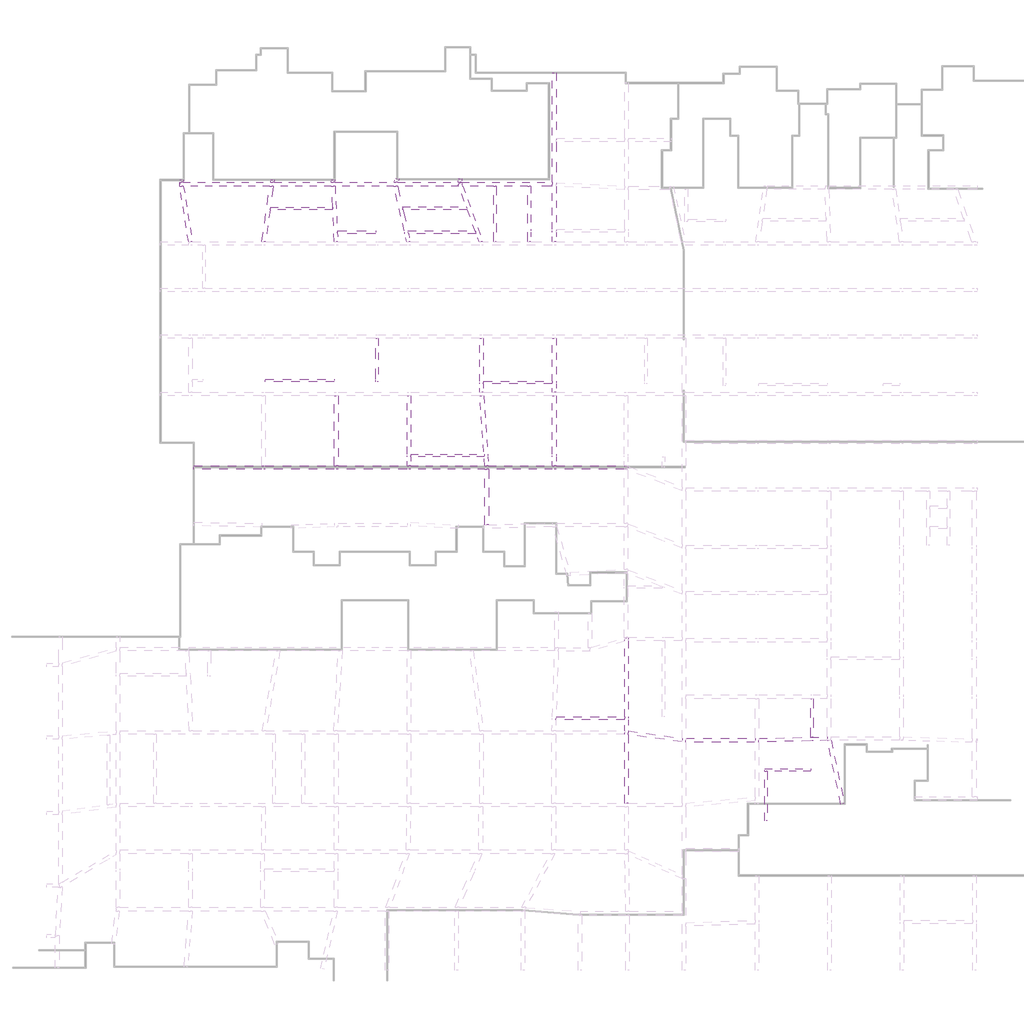
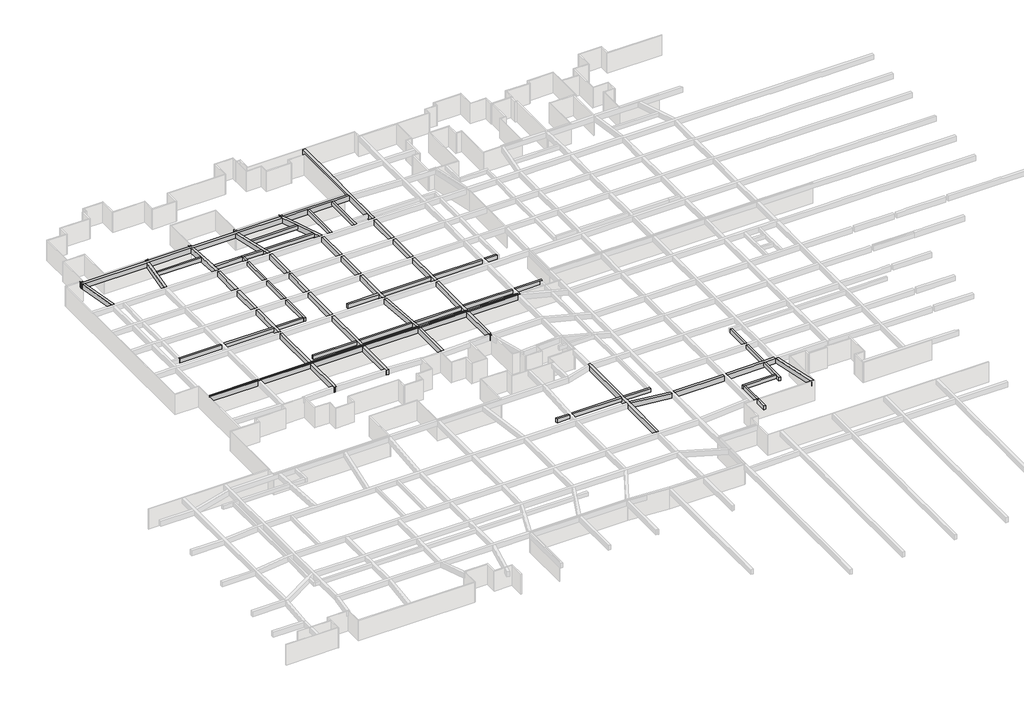
# One storey, part 12 of 16: 40 beams.
"""IFC4 building model written with IfcOpenShell, lengths in millimetres."""

from ifc_helpers import new_model, si_unit, frame, origin, place, context, project, spatial, polyline, outline, extrude, faceted_brep, element, save

model = new_model("IFC4")

# Units and contexts
model_context = context("Model", 3, world=origin())
ifc_project = project(units=[si_unit("LENGTHUNIT", "METRE", prefix="MILLI")], contexts=[model_context])

# Site, building, storey
site = spatial("IfcSite", under=ifc_project)
building = spatial("IfcBuilding", under=site)
storey = spatial("IfcBuildingStorey", under=building, Name="户型图", Elevation=0.0)

# Beams
placement = place(None, origin())
element("IfcBeam", 1, ObjectType="混凝土 - 矩形梁 : KL_beam", at=placement, inside=storey, context=model_context, shape_type="Brep", body=[
    faceted_brep([(86828.9386535, 165312.5884701, 3300.0), (86828.9386535, 165312.5884701, 2500.0), (86828.9386535, 164912.5884701, 2500.0), (86828.9386535, 164912.5884701, 3300.0), (94416.2109037, 164912.5884701, 3300.0), (94816.2109037, 164912.5884701, 3300.0), (102516.2109037, 164912.5884701, 3300.0), (102916.2109037, 164912.5884701, 3300.0), (110616.2109037, 164912.5884701, 3300.0), (111016.2109037, 164912.5884701, 3300.0), (119289.6107616, 164912.5884701, 3300.0), (119689.6107616, 164912.5884701, 3300.0), (126816.2109037, 164912.5884701, 3300.0), (127216.2109037, 164912.5884701, 3300.0), (134828.9386535, 164912.5884701, 3300.0), (134991.8708445, 164912.5884701, 3300.0), (135228.9386535, 164912.5884701, 3300.0), (135228.9386535, 165250.0446618, 3300.0), (135216.2109037, 165254.9303872, 3300.0), (135066.0064625, 165312.5884701, 3300.0), (134816.2109037, 165312.5884701, 3300.0), (127216.2109037, 165312.5884701, 3300.0), (126816.2109037, 165312.5884701, 3300.0), (119676.1137788, 165312.5884701, 3300.0), (119275.1370196, 165312.5884701, 3300.0), (111016.2109037, 165312.5884701, 3300.0), (110616.2109037, 165312.5884701, 3300.0), (102916.2109037, 165312.5884701, 3300.0), (102516.2109037, 165312.5884701, 3300.0), (94816.2109037, 165312.5884701, 3300.0), (94416.2109037, 165312.5884701, 3300.0), (94416.2109037, 164912.5884701, 2500.0), (94816.2109037, 164912.5884701, 2500.0), (102516.2109037, 164912.5884701, 2500.0), (102916.2109037, 164912.5884701, 2500.0), (110616.2109037, 164912.5884701, 2500.0), (111016.2109037, 164912.5884701, 2500.0), (119289.6107616, 164912.5884701, 2500.0), (119689.6107616, 164912.5884701, 2500.0), (126816.2109037, 164912.5884701, 2500.0), (127216.2109037, 164912.5884701, 2500.0), (134828.9386535, 164912.5884701, 2500.0), (134991.8708445, 164912.5884701, 2500.0), (135228.9386535, 164912.5884701, 2500.0), (94416.2109037, 165312.5884701, 2500.0), (94816.2109037, 165312.5884701, 2500.0), (102516.2109037, 165312.5884701, 2500.0), (102916.2109037, 165312.5884701, 2500.0), (110616.2109037, 165312.5884701, 2500.0), (111016.2109037, 165312.5884701, 2500.0), (119275.1370196, 165312.5884701, 2500.0), (119676.1137788, 165312.5884701, 2500.0), (126816.2109037, 165312.5884701, 2500.0), (127216.2109037, 165312.5884701, 2500.0), (134816.2109037, 165312.5884701, 2500.0), (135066.0064625, 165312.5884701, 2500.0), (135216.2109037, 165254.9303872, 2500.0), (135228.9386535, 165250.0446618, 2500.0)], [[[0, 1, 2, 3]], [[0, 3, 4, 5, 6, 7, 8, 9, 10, 11, 12, 13, 14, 15, 16, 17, 18, 19, 20, 21, 22, 23, 24, 25, 26, 27, 28, 29, 30]], [[3, 2, 31, 32, 33, 34, 35, 36, 37, 38, 39, 40, 41, 42, 43, 16, 15, 14, 13, 12, 11, 10, 9, 8, 7, 6, 5, 4]], [[2, 1, 44, 45, 46, 47, 48, 49, 50, 51, 52, 53, 54, 55, 56, 57, 43, 42, 41, 40, 39, 38, 37, 36, 35, 34, 33, 32, 31]], [[1, 0, 30, 29, 28, 27, 26, 25, 24, 23, 22, 21, 20, 19, 55, 54, 53, 52, 51, 50, 49, 48, 47, 46, 45, 44]], [[17, 57, 56, 55, 19, 18]], [[57, 17, 16, 43]]]),
])
element("IfcBeam", 2, ObjectType="混凝土 - 矩形梁 : KL_beam", at=placement, inside=storey, context=model_context, shape_type="Brep", body=[
    faceted_brep([(102916.2109037, 189895.7397162, 3300.0), (102516.2109037, 189895.7397162, 3300.0), (102516.2109037, 185072.5884701, 3300.0), (102916.2109037, 185072.5884701, 3300.0), (102516.2109037, 189895.7397162, 2500.0), (102516.2109037, 185072.5884701, 2500.0), (102916.2109037, 189895.7397162, 2500.0), (102916.2109037, 185072.5884701, 2500.0)], [[[0, 1, 2, 3]], [[1, 4, 5, 2]], [[4, 6, 7, 5]], [[6, 0, 3, 7]], [[1, 0, 6, 4]], [[3, 2, 5, 7]]]),
    faceted_brep([(102516.2109037, 184672.5884701, 3300.0), (102916.2109037, 184672.5884701, 3300.0), (102916.2109037, 184672.5884701, 2500.0), (102516.2109037, 184672.5884701, 2500.0), (102916.2109037, 179912.5884701, 3300.0), (102516.2109037, 179912.5884701, 3300.0), (102516.2109037, 179912.5884701, 2500.0), (102916.2109037, 179912.5884701, 2500.0)], [[[0, 1, 2, 3]], [[4, 5, 6, 7]], [[1, 0, 5, 4]], [[0, 3, 6, 5]], [[3, 2, 7, 6]], [[2, 1, 4, 7]]]),
    faceted_brep([(102916.2109037, 173512.5884701, 3300.0), (102916.2109037, 174669.5403425, 3300.0), (102916.2109037, 174969.5403425, 3300.0), (102916.2109037, 179512.5884701, 3300.0), (102516.2109037, 179512.5884701, 3300.0), (102516.2109037, 174969.5403425, 3300.0), (102516.2109037, 174669.5403425, 3300.0), (102516.2109037, 173512.5884701, 3300.0), (102516.2109037, 179512.5884701, 2500.0), (102516.2109037, 173512.5884701, 2500.0), (102916.2109037, 179512.5884701, 2500.0), (102916.2109037, 173512.5884701, 2500.0)], [[[0, 1, 2, 3, 4, 5, 6, 7]], [[7, 6, 5, 4, 8, 9]], [[9, 8, 10, 11]], [[3, 2, 1, 0, 11, 10]], [[4, 3, 10, 8]], [[0, 7, 9, 11]]]),
    faceted_brep([(102516.2109037, 173112.5884701, 3300.0), (102916.2109037, 173112.5884701, 3300.0), (102916.2109037, 173112.5884701, 2500.0), (102516.2109037, 173112.5884701, 2500.0), (102916.2109037, 165312.5884701, 3300.0), (102516.2109037, 165312.5884701, 3300.0), (102516.2109037, 165312.5884701, 2500.0), (102916.2109037, 165312.5884701, 2500.0)], [[[0, 1, 2, 3]], [[4, 5, 6, 7]], [[1, 0, 5, 4]], [[0, 3, 6, 5]], [[3, 2, 7, 6]], [[2, 1, 4, 7]]]),
    faceted_brep([(102516.2109037, 164912.5884701, 3300.0), (102916.2109037, 164912.5884701, 3300.0), (102916.2109037, 164912.5884701, 2500.0), (102516.2109037, 164912.5884701, 2500.0), (102916.2109037, 158502.9404881, 3300.0), (102719.8772917, 158495.7397162, 3300.0), (102516.2109037, 158488.2700059, 3300.0), (102516.2109037, 158488.2700059, 2500.0), (102719.8772917, 158495.7397162, 2500.0), (102916.2109037, 158502.9404881, 2500.0), (102916.2109037, 158895.7397162, 3300.0), (102516.2109037, 158888.5389443, 3300.0), (102516.2109037, 158888.5389443, 2500.0), (102916.2109037, 158895.7397162, 2500.0)], [[[0, 1, 2, 3]], [[4, 5, 6, 7, 8, 9]], [[6, 5, 4, 10, 1, 0, 11]], [[7, 6, 11, 0, 3, 12]], [[9, 8, 7, 12, 3, 2, 13]], [[4, 9, 13, 2, 1, 10]]]),
])
element("IfcBeam", 3, ObjectType="混凝土 - 矩形梁 : KL_beam", at=placement, inside=storey, context=model_context, shape_type="Brep", body=[
    faceted_brep([(111016.2109037, 189895.7397162, 3300.0), (110616.2109037, 189895.7397162, 3300.0), (110616.2109037, 185072.5884701, 3300.0), (111016.2109037, 185072.5884701, 3300.0), (110616.2109037, 189895.7397162, 2500.0), (110616.2109037, 185072.5884701, 2500.0), (111016.2109037, 189895.7397162, 2500.0), (111016.2109037, 185072.5884701, 2500.0)], [[[0, 1, 2, 3]], [[1, 4, 5, 2]], [[4, 6, 7, 5]], [[6, 0, 3, 7]], [[1, 0, 6, 4]], [[3, 2, 5, 7]]]),
    faceted_brep([(110616.2109037, 184672.5884701, 3300.0), (111016.2109037, 184672.5884701, 3300.0), (111016.2109037, 184672.5884701, 2500.0), (110616.2109037, 184672.5884701, 2500.0), (111016.2109037, 179912.5884701, 3300.0), (110616.2109037, 179912.5884701, 3300.0), (110616.2109037, 179912.5884701, 2500.0), (111016.2109037, 179912.5884701, 2500.0)], [[[0, 1, 2, 3]], [[4, 5, 6, 7]], [[1, 0, 5, 4]], [[0, 3, 6, 5]], [[3, 2, 7, 6]], [[2, 1, 4, 7]]]),
    faceted_brep([(111016.2109037, 179512.5884701, 3300.0), (110616.2109037, 179512.5884701, 3300.0), (110616.2109037, 173512.5884701, 3300.0), (111016.2109037, 173512.5884701, 3300.0), (110616.2109037, 179512.5884701, 2500.0), (110616.2109037, 173512.5884701, 2500.0), (111016.2109037, 179512.5884701, 2500.0), (111016.2109037, 173512.5884701, 2500.0)], [[[0, 1, 2, 3]], [[1, 4, 5, 2]], [[4, 6, 7, 5]], [[6, 0, 3, 7]], [[1, 0, 6, 4]], [[3, 2, 5, 7]]]),
    faceted_brep([(110616.2109037, 173112.5884701, 3300.0), (111016.2109037, 173112.5884701, 3300.0), (111016.2109037, 173112.5884701, 2500.0), (110616.2109037, 173112.5884701, 2500.0), (111016.2109037, 165312.5884701, 3300.0), (110616.2109037, 165312.5884701, 3300.0), (110616.2109037, 165312.5884701, 2500.0), (111016.2109037, 165312.5884701, 2500.0), (110616.2109037, 166595.0298489, 3300.0), (110616.2109037, 166295.0298489, 3300.0), (111016.2109037, 166295.0298489, 3300.0), (111016.2109037, 166595.0298489, 3300.0)], [[[0, 1, 2, 3]], [[4, 5, 6, 7]], [[1, 0, 8, 9, 5, 4, 10, 11]], [[0, 3, 6, 5, 9, 8]], [[3, 2, 7, 6]], [[2, 1, 11, 10, 4, 7]]]),
    faceted_brep([(110616.2109037, 164912.5884701, 3300.0), (111016.2109037, 164912.5884701, 3300.0), (111016.2109037, 164912.5884701, 2500.0), (110616.2109037, 164912.5884701, 2500.0), (111016.2109037, 158495.7397162, 3300.0), (110616.2109037, 158495.7397162, 3300.0), (110616.2109037, 158495.7397162, 2500.0), (111016.2109037, 158495.7397162, 2500.0), (111016.2109037, 158585.1907676, 3300.0), (111016.2109037, 158985.7192923, 3300.0), (110616.2109037, 158895.7397162, 3300.0), (110616.2109037, 158895.7397162, 2500.0), (111016.2109037, 158985.7192923, 2500.0), (111016.2109037, 158585.1907676, 2500.0)], [[[0, 1, 2, 3]], [[4, 5, 6, 7]], [[5, 4, 8, 9, 1, 0, 10]], [[6, 5, 10, 0, 3, 11]], [[7, 6, 11, 3, 2, 12, 13]], [[4, 7, 13, 12, 2, 1, 9, 8]]]),
])
element("IfcBeam", 4, ObjectType="混凝土 - 矩形梁 : KL_beam", at=placement, inside=storey, context=model_context, shape_type="Brep", body=[
    faceted_brep([(118716.2109037, 173512.5884701, 3300.0), (119116.2109037, 173512.5884701, 3300.0), (119116.2109037, 174424.6482986, 3300.0), (119116.2109037, 174724.6482986, 3300.0), (119116.2109037, 179512.5884701, 3300.0), (118716.2109037, 179512.5884701, 3300.0), (118716.2109037, 174724.6482986, 3300.0), (118716.2109037, 174424.6482986, 3300.0), (118716.2109037, 173512.5884701, 2500.0), (118716.2109037, 179512.5884701, 2500.0), (119116.2109037, 173512.5884701, 2500.0), (119116.2109037, 179512.5884701, 2500.0)], [[[0, 1, 2, 3, 4, 5, 6, 7]], [[8, 0, 7, 6, 5, 9]], [[10, 8, 9, 11]], [[1, 10, 11, 4, 3, 2]], [[1, 0, 8, 10]], [[5, 4, 11, 9]]]),
    faceted_brep([(118716.2109037, 189895.7397162, 3300.0), (119116.2109037, 189895.7397162, 3300.0), (119116.2109037, 189895.7397162, 2500.0), (118716.2109037, 189895.7397162, 2500.0), (119116.2109037, 185072.5884701, 3300.0), (118716.2109037, 185072.5884701, 3300.0), (118716.2109037, 185072.5884701, 2500.0), (119116.2109037, 185072.5884701, 2500.0)], [[[0, 1, 2, 3]], [[4, 5, 6, 7]], [[1, 0, 5, 4]], [[0, 3, 6, 5]], [[3, 2, 7, 6]], [[2, 1, 4, 7]]]),
    faceted_brep([(118716.2109037, 184672.5884701, 3300.0), (119116.2109037, 184672.5884701, 3300.0), (119116.2109037, 184672.5884701, 2500.0), (118716.2109037, 184672.5884701, 2500.0), (119116.2109037, 179912.5884701, 3300.0), (118716.2109037, 179912.5884701, 3300.0), (118716.2109037, 179912.5884701, 2500.0), (119116.2109037, 179912.5884701, 2500.0)], [[[0, 1, 2, 3]], [[4, 5, 6, 7]], [[1, 0, 5, 4]], [[0, 3, 6, 5]], [[3, 2, 7, 6]], [[2, 1, 4, 7]]]),
])
element("IfcBeam", 5, ObjectType="混凝土 - 矩形梁 : KL_beam", at=placement, inside=storey, context=model_context, shape_type="Brep", body=[
    faceted_brep([(126816.2109037, 173512.5884701, 3300.0), (127216.2109037, 173512.5884701, 3300.0), (127216.2109037, 174424.6482986, 3300.0), (127216.2109037, 174724.6482986, 3300.0), (127216.2109037, 179512.5884701, 3300.0), (126816.2109037, 179512.5884701, 3300.0), (126816.2109037, 174724.6482986, 3300.0), (126816.2109037, 174424.6482986, 3300.0), (126816.2109037, 173512.5884701, 2500.0), (126816.2109037, 179512.5884701, 2500.0), (127216.2109037, 173512.5884701, 2500.0), (127216.2109037, 179512.5884701, 2500.0)], [[[0, 1, 2, 3, 4, 5, 6, 7]], [[8, 0, 7, 6, 5, 9]], [[10, 8, 9, 11]], [[1, 10, 11, 4, 3, 2]], [[1, 0, 8, 10]], [[5, 4, 11, 9]]]),
    faceted_brep([(126816.2109037, 189895.7397162, 3300.0), (127216.2109037, 189895.7397162, 3300.0), (127216.2109037, 189895.7397162, 2500.0), (126816.2109037, 189895.7397162, 2500.0), (127216.2109037, 185072.5884701, 3300.0), (126816.2109037, 185072.5884701, 3300.0), (126816.2109037, 185072.5884701, 2500.0), (127216.2109037, 185072.5884701, 2500.0)], [[[0, 1, 2, 3]], [[4, 5, 6, 7]], [[1, 0, 5, 4]], [[0, 3, 6, 5]], [[3, 2, 7, 6]], [[2, 1, 4, 7]]]),
    faceted_brep([(126816.2109037, 184672.5884701, 3300.0), (127216.2109037, 184672.5884701, 3300.0), (127216.2109037, 184672.5884701, 2500.0), (126816.2109037, 184672.5884701, 2500.0), (127216.2109037, 179912.5884701, 3300.0), (126816.2109037, 179912.5884701, 3300.0), (126816.2109037, 179912.5884701, 2500.0), (127216.2109037, 179912.5884701, 2500.0)], [[[0, 1, 2, 3]], [[4, 5, 6, 7]], [[1, 0, 5, 4]], [[0, 3, 6, 5]], [[3, 2, 7, 6]], [[2, 1, 4, 7]]]),
])
element("IfcBeam", 6, ObjectType="混凝土 - 矩形梁 : KL_beam", at=placement, inside=storey, context=model_context, shape_type="Brep", body=[
    faceted_brep([(127216.2109037, 173112.5884701, 3300.0), (126816.2109037, 173112.5884701, 3300.0), (126816.2109037, 166595.0298489, 3300.0), (126816.2109037, 166295.0298489, 3300.0), (126816.2109037, 165312.5884701, 3300.0), (127216.2109037, 165312.5884701, 3300.0), (127216.2109037, 166295.0298489, 3300.0), (127216.2109037, 166595.0298489, 3300.0), (126816.2109037, 173112.5884701, 2500.0), (126816.2109037, 165312.5884701, 2500.0), (127216.2109037, 173112.5884701, 2500.0), (127216.2109037, 165312.5884701, 2500.0)], [[[0, 1, 2, 3, 4, 5, 6, 7]], [[1, 8, 9, 4, 3, 2]], [[8, 10, 11, 9]], [[10, 0, 7, 6, 5, 11]], [[1, 0, 10, 8]], [[5, 4, 9, 11]]]),
    faceted_brep([(126816.2109037, 164912.5884701, 3300.0), (127216.2109037, 164912.5884701, 3300.0), (127216.2109037, 164912.5884701, 2500.0), (126816.2109037, 164912.5884701, 2500.0), (126816.2109037, 158509.867597, 3300.0), (126866.6192101, 158511.1605747, 3300.0), (127018.7754912, 158515.0633975, 3300.0), (127216.2109037, 158520.1276342, 3300.0), (127216.2109037, 158915.0633975, 3300.0), (126816.2109037, 158909.9991608, 3300.0), (126816.2109037, 158509.867597, 2500.0), (126816.2109037, 158909.9991608, 2500.0), (127216.2109037, 158520.1276342, 2500.0), (127018.7754912, 158515.0633975, 2500.0), (126866.6192101, 158511.1605747, 2500.0), (127216.2109037, 158915.0633975, 2500.0)], [[[0, 1, 2, 3]], [[4, 5, 6, 7, 8, 1, 0, 9]], [[10, 4, 9, 0, 3, 11]], [[12, 13, 14, 10, 11, 3, 2, 15]], [[7, 12, 15, 2, 1, 8]], [[7, 6, 5, 4, 10, 14, 13, 12]]]),
])
element("IfcBeam", 7, ObjectType="混凝土 - 矩形梁 : KL_beam", at=placement, inside=storey, context=model_context, shape_type="Brep", body=[
    faceted_brep([(119130.6846457, 173112.5884701, 3300.0), (118729.7078864, 173112.5884701, 3300.0), (119185.4599825, 166595.0298489, 3300.0), (119206.4380261, 166295.0298489, 3300.0), (119275.1370196, 165312.5884701, 3300.0), (119676.1137788, 165312.5884701, 3300.0), (119607.4147853, 166295.0298489, 3300.0), (119586.4367417, 166595.0298489, 3300.0), (118729.7078864, 173112.5884701, 2500.0), (119275.1370196, 165312.5884701, 2500.0), (119130.6846457, 173112.5884701, 2500.0), (119676.1137788, 165312.5884701, 2500.0)], [[[0, 1, 2, 3, 4, 5, 6, 7]], [[1, 8, 9, 4, 3, 2]], [[8, 10, 11, 9]], [[10, 0, 7, 6, 5, 11]], [[1, 0, 10, 8]], [[5, 4, 9, 11]]]),
])
element("IfcBeam", 8, ObjectType="混凝土 - 矩形梁 : KL_beam", at=placement, inside=storey, context=model_context, shape_type="Brep", body=[
    faceted_brep([(126816.2109037, 209112.7856546, 3300.0), (127216.2109037, 209112.7856546, 3300.0), (127216.2109037, 209112.7856546, 2500.0), (126816.2109037, 209112.7856546, 2500.0), (126816.2109037, 196873.5880617, 3300.0), (126816.2109037, 196473.5880617, 3300.0), (126816.2109037, 191637.5884701, 3300.0), (126816.2109037, 191337.5884701, 3300.0), (126816.2109037, 190295.7397162, 3300.0), (127216.2109037, 190295.7397162, 3300.0), (127216.2109037, 191337.5884701, 3300.0), (127216.2109037, 191637.5884701, 3300.0), (127216.2109037, 196462.8320366, 3300.0), (127216.2109037, 196863.380975, 3300.0), (127216.2109037, 201412.9009701, 3300.0), (127216.2109037, 201812.9009701, 3300.0), (127216.2109037, 190295.7397162, 2500.0), (127216.2109037, 196462.8320366, 2500.0), (127216.2109037, 196863.380975, 2500.0), (127216.2109037, 201412.9009701, 2500.0), (127216.2109037, 201812.9009701, 2500.0), (126816.2109037, 190295.7397162, 2500.0), (126816.2109037, 196473.5880617, 2500.0), (126816.2109037, 196873.5880617, 2500.0)], [[[0, 1, 2, 3]], [[1, 0, 4, 5, 6, 7, 8, 9, 10, 11, 12, 13, 14, 15]], [[2, 1, 15, 14, 13, 12, 11, 10, 9, 16, 17, 18, 19, 20]], [[3, 2, 20, 19, 18, 17, 16, 21, 22, 23]], [[0, 3, 23, 22, 21, 8, 7, 6, 5, 4]], [[9, 8, 21, 16]]]),
])
element("IfcBeam", 9, ObjectType="混凝土 - 矩形梁 : KL_beam", at=placement, inside=storey, context=model_context, shape_type="Brep", body=[
    faceted_brep([(116662.111408, 196873.5880617, 3300.0), (116286.2343597, 196736.7800043, 3300.0), (116382.0283927, 196473.5880617, 3300.0), (117225.8528022, 194155.1995507, 3300.0), (117335.0438725, 193855.1995507, 3300.0), (118203.3528134, 191469.5403425, 3300.0), (118312.5438836, 191169.5403425, 3300.0), (118630.5813023, 190295.7397162, 3300.0), (119056.2524113, 190295.7397162, 3300.0), (116807.6995017, 196473.5880617, 3300.0), (116662.111408, 196873.5880617, 2500.0), (119056.2524113, 190295.7397162, 2500.0), (116807.6995017, 196473.5880617, 2500.0), (116286.2343597, 196736.7800043, 2500.0), (118630.5813023, 190295.7397162, 2500.0), (116382.0283927, 196473.5880617, 2500.0)], [[[0, 1, 2, 3, 4, 5, 6, 7, 8, 9]], [[10, 0, 9, 8, 11, 12]], [[13, 10, 12, 11, 14, 15]], [[1, 13, 15, 14, 7, 6, 5, 4, 3, 2]], [[8, 7, 14, 11]], [[1, 0, 10, 13]]]),
])
element("IfcBeam", 10, ObjectType="混凝土 - 矩形梁 : KL_beam", at=placement, inside=storey, context=model_context, shape_type="Brep", body=[
    faceted_brep([(116662.111408, 196873.5880617, 3300.0), (116807.6995017, 196473.5880617, 3300.0), (120273.9609037, 196473.5880617, 3300.0), (120573.9609037, 196473.5880617, 3300.0), (124073.9303911, 196473.5880617, 3300.0), (124373.9303911, 196473.5880617, 3300.0), (126816.2109037, 196473.5880617, 3300.0), (126816.2109037, 196873.5880617, 3300.0), (116722.0699004, 196873.5880617, 3300.0), (116807.6995017, 196473.5880617, 2500.0), (126816.2109037, 196473.5880617, 2500.0), (116662.111408, 196873.5880617, 2500.0), (116722.0699004, 196873.5880617, 2500.0), (126816.2109037, 196873.5880617, 2500.0)], [[[0, 1, 2, 3, 4, 5, 6, 7, 8]], [[1, 9, 10, 6, 5, 4, 3, 2]], [[9, 11, 12, 13, 10]], [[11, 0, 8, 7, 13, 12]], [[1, 0, 11, 9]], [[7, 6, 10, 13]]]),
])
element("IfcBeam", 11, ObjectType="混凝土 - 矩形梁 : KL_beam", at=placement, inside=storey, context=model_context, shape_type="Brep", body=[
    faceted_brep([(110564.7764439, 190295.7397162, 3300.0), (110975.298087, 190295.7397162, 3300.0), (110773.565317, 191169.5403425, 3300.0), (110704.3048596, 191469.5403425, 3300.0), (110153.5320336, 193855.1995507, 3300.0), (110084.2715763, 194155.1995507, 3300.0), (109549.0294144, 196473.5880617, 3300.0), (109138.5077713, 196473.5880617, 3300.0), (110293.7832165, 191469.5403425, 3300.0), (110363.0436739, 191169.5403425, 3300.0), (110975.298087, 190295.7397162, 2500.0), (109549.0294144, 196473.5880617, 2500.0), (110564.7764439, 190295.7397162, 2500.0), (109138.5077713, 196473.5880617, 2500.0)], [[[0, 1, 2, 3, 4, 5, 6, 7, 8, 9]], [[1, 10, 11, 6, 5, 4, 3, 2]], [[10, 12, 13, 11]], [[12, 0, 9, 8, 7, 13]], [[1, 0, 12, 10]], [[7, 6, 11, 13]]]),
])
element("IfcBeam", 12, ObjectType="混凝土 - 矩形梁 : KL_beam", at=placement, inside=storey, context=model_context, shape_type="Brep", body=[
    faceted_brep([(116382.0283927, 196473.5880617, 3300.0), (116286.2343597, 196736.7800043, 3300.0), (116662.111408, 196873.5880617, 3300.0), (116322.0699004, 196873.5880617, 3300.0), (109583.224556, 196873.5880617, 3300.0), (109157.553447, 196873.5880617, 3300.0), (102571.4804794, 196873.5880617, 3300.0), (102171.4804794, 196873.5880617, 3300.0), (95823.9296537, 196873.5880617, 3300.0), (95423.9296537, 196873.5880617, 3300.0), (85652.3327458, 196873.5880617, 3300.0), (85281.5166087, 196873.5880617, 3300.0), (85281.5166087, 196473.5880617, 3300.0), (85686.502659, 196473.5880617, 3300.0), (95310.5935192, 196473.5880617, 3300.0), (95714.5245482, 196473.5880617, 3300.0), (102181.6875661, 196473.5880617, 3300.0), (102582.2365045, 196473.5880617, 3300.0), (109138.5077713, 196473.5880617, 3300.0), (109549.0294144, 196473.5880617, 3300.0), (85281.5166087, 196873.5880617, 2500.0), (116662.111408, 196873.5880617, 2500.0), (116322.0699004, 196873.5880617, 2500.0), (109583.224556, 196873.5880617, 2500.0), (109157.553447, 196873.5880617, 2500.0), (102571.4804794, 196873.5880617, 2500.0), (102171.4804794, 196873.5880617, 2500.0), (95823.9296537, 196873.5880617, 2500.0), (95423.9296537, 196873.5880617, 2500.0), (85652.3327458, 196873.5880617, 2500.0), (116286.2343597, 196736.7800043, 2500.0), (116382.0283927, 196473.5880617, 2500.0), (109549.0294144, 196473.5880617, 2500.0), (109138.5077713, 196473.5880617, 2500.0), (102582.2365045, 196473.5880617, 2500.0), (102181.6875661, 196473.5880617, 2500.0), (95714.5245482, 196473.5880617, 2500.0), (95310.5935192, 196473.5880617, 2500.0), (85686.502659, 196473.5880617, 2500.0), (85281.5166087, 196473.5880617, 2500.0)], [[[0, 1, 2, 3, 4, 5, 6, 7, 8, 9, 10, 11, 12, 13, 14, 15, 16, 17, 18, 19]], [[20, 11, 10, 9, 8, 7, 6, 5, 4, 3, 2, 21, 22, 23, 24, 25, 26, 27, 28, 29]], [[30, 31, 32, 33, 34, 35, 36, 37, 38, 39, 20, 29, 28, 27, 26, 25, 24, 23, 22, 21]], [[31, 0, 19, 18, 17, 16, 15, 14, 13, 12, 39, 38, 37, 36, 35, 34, 33, 32]], [[1, 0, 31, 30]], [[12, 11, 20, 39]], [[1, 30, 21, 2]]]),
])
element("IfcBeam", 13, ObjectType="混凝土 - 矩形梁 : KL_beam", at=placement, inside=storey, context=model_context, shape_type="Brep", body=[
    faceted_brep([(94442.3535561, 190295.7397162, 3300.0), (94846.2845851, 190295.7397162, 3300.0), (95341.1878431, 193817.1593735, 3300.0), (95383.3500935, 194117.1593735, 3300.0), (95714.5245482, 196473.5880617, 3300.0), (95310.5935192, 196473.5880617, 3300.0), (94846.2845851, 190295.7397162, 2500.0), (95714.5245482, 196473.5880617, 2500.0), (94442.3535561, 190295.7397162, 2500.0), (95310.5935192, 196473.5880617, 2500.0)], [[[0, 1, 2, 3, 4, 5]], [[1, 6, 7, 4, 3, 2]], [[6, 8, 9, 7]], [[8, 0, 5, 9]], [[1, 0, 8, 6]], [[5, 4, 7, 9]]]),
])
element("IfcBeam", 14, ObjectType="混凝土 - 矩形梁 : KL_beam", at=placement, inside=storey, context=model_context, shape_type="Brep", body=[
    faceted_brep([(102505.4548786, 190295.7397162, 3300.0), (102906.003817, 190295.7397162, 3300.0), (102860.2098666, 191169.5403425, 3300.0), (102844.4875329, 191469.5403425, 3300.0), (102582.2365045, 196473.5880617, 3300.0), (102181.6875661, 196473.5880617, 3300.0), (102305.1827607, 194117.1593735, 3300.0), (102320.9050944, 193817.1593735, 3300.0), (102906.003817, 190295.7397162, 2500.0), (102582.2365045, 196473.5880617, 2500.0), (102505.4548786, 190295.7397162, 2500.0), (102181.6875661, 196473.5880617, 2500.0)], [[[0, 1, 2, 3, 4, 5, 6, 7]], [[1, 8, 9, 4, 3, 2]], [[8, 10, 11, 9]], [[10, 0, 7, 6, 5, 11]], [[1, 0, 10, 8]], [[5, 4, 9, 11]]]),
])
element("IfcBeam", 15, ObjectType="混凝土 - 矩形梁 : KL_beam", at=placement, inside=storey, context=model_context, shape_type="Brep", body=[
    faceted_brep([(86259.9916613, 190295.7397162, 3300.0), (86294.1615746, 190295.7397162, 3300.0), (86664.9777116, 190295.7397162, 3300.0), (85686.502659, 196473.5880617, 3300.0), (85281.5166087, 196473.5880617, 3300.0), (86664.9777116, 190295.7397162, 2500.0), (85686.502659, 196473.5880617, 2500.0), (86294.1615746, 190295.7397162, 2500.0), (86259.9916613, 190295.7397162, 2500.0), (85281.5166087, 196473.5880617, 2500.0)], [[[0, 1, 2, 3, 4]], [[2, 5, 6, 3]], [[5, 7, 8, 9, 6]], [[8, 0, 4, 9]], [[5, 2, 1, 0, 8, 7]], [[4, 3, 6, 9]]]),
])
element("IfcBeam", 16, ObjectType="混凝土 - 矩形梁 : KL_beam", at=placement, inside=storey, context=model_context, shape_type="Brep", body=[
    faceted_brep([(85252.3327458, 197173.5880617, 3300.0), (85652.3327458, 197173.5880617, 3300.0), (85652.3327458, 197173.5880617, 2500.0), (85252.3327458, 197173.5880617, 2500.0), (85252.3327458, 196657.8477203, 3300.0), (85281.5166087, 196473.5880617, 3300.0), (85281.5166087, 196873.5880617, 3300.0), (85623.1488829, 196873.5880617, 3300.0), (85652.3327458, 196873.5880617, 3300.0), (85652.3327458, 196873.5880617, 2500.0), (85623.1488829, 196873.5880617, 2500.0), (85281.5166087, 196873.5880617, 2500.0), (85281.5166087, 196473.5880617, 2500.0), (85252.3327458, 196657.8477203, 2500.0)], [[[0, 1, 2, 3]], [[1, 0, 4, 5, 6, 7, 8]], [[2, 1, 8, 9]], [[3, 2, 9, 10, 11, 12, 13]], [[0, 3, 13, 4]], [[5, 4, 13, 12]], [[6, 11, 10, 9, 8, 7]], [[11, 6, 5, 12]]]),
])
element("IfcBeam", 17, ObjectType="混凝土 - 矩形梁 : KL_beam", at=placement, inside=storey, context=model_context, shape_type="SweptSolid", body=[
    extrude(outline(polyline([(95423.9296537, 197162.7132659), (95823.9296537, 197162.7132659), (95823.9296537, 196873.5880617), (95423.9296537, 196873.5880617), (95423.9296537, 197162.7132659)])), frame((0.0, 0.0, 2500.0), z_axis=(0.0, 0.0, 1.0), x_axis=(1.0, 0.0, 0.0)), (0.0, 0.0, 1.0), 800.0),
])
element("IfcBeam", 18, ObjectType="混凝土 - 矩形梁 : KL_beam", at=placement, inside=storey, context=model_context, shape_type="SweptSolid", body=[
    extrude(outline(polyline([(102171.4804794, 197162.7132659), (102571.4804794, 197162.7132659), (102571.4804794, 196873.5880617), (102171.4804794, 196873.5880617), (102171.4804794, 197162.7132659)])), frame((0.0, 0.0, 2500.0), z_axis=(0.0, 0.0, 1.0), x_axis=(1.0, 0.0, 0.0)), (0.0, 0.0, 1.0), 800.0),
])
element("IfcBeam", 19, ObjectType="混凝土 - 矩形梁 : KL_beam", at=placement, inside=storey, context=model_context, shape_type="SweptSolid", body=[
    extrude(outline(polyline([(109335.8848749, 197363.5496329), (109711.7619232, 197226.7415756), (109583.224556, 196873.5880617), (109157.553447, 196873.5880617), (109335.8848749, 197363.5496329)])), frame((0.0, 0.0, 2500.0), z_axis=(0.0, 0.0, 1.0), x_axis=(1.0, 0.0, 0.0)), (0.0, 0.0, 1.0), 800.0),
])
element("IfcBeam", 20, ObjectType="混凝土 - 矩形梁 : KL_beam", at=placement, inside=storey, context=model_context, shape_type="Brep", body=[
    faceted_brep([(116322.0699004, 197262.7098479, 3300.0), (116722.0699004, 197262.7098479, 3300.0), (116722.0699004, 197262.7098479, 2500.0), (116322.0699004, 197262.7098479, 2500.0), (116322.0699004, 196873.5880617, 3300.0), (116662.111408, 196873.5880617, 3300.0), (116722.0699004, 196873.5880617, 3300.0), (116722.0699004, 196873.5880617, 2500.0), (116662.111408, 196873.5880617, 2500.0), (116322.0699004, 196873.5880617, 2500.0)], [[[0, 1, 2, 3]], [[1, 0, 4, 5, 6]], [[2, 1, 6, 7]], [[3, 2, 7, 8, 9]], [[0, 3, 9, 4]], [[4, 9, 8, 7, 6, 5]]]),
])
element("IfcBeam", 21, ObjectType="混凝土 - 矩形梁 : KL_beam", at=placement, inside=storey, context=model_context, shape_type="SweptSolid", body=[
    extrude(outline(polyline([(119289.6107616, 164912.5884701), (119689.6107616, 164912.5884701), (119689.6107616, 158727.2012041), (119289.6107616, 158716.9411668), (119289.6107616, 164912.5884701)])), frame((0.0, 0.0, 2500.0), z_axis=(0.0, 0.0, 1.0), x_axis=(1.0, 0.0, 0.0)), (0.0, 0.0, 1.0), 800.0),
])
element("IfcBeam", 22, ObjectType="混凝土 - 矩形梁 : KL_beam", at=placement, inside=storey, context=model_context, shape_type="SweptSolid", body=[
    extrude(outline(polyline([(141666.2091209, 134512.5884701), (141666.2091209, 134912.5884701), (149416.2109037, 134912.5884701), (149416.2109037, 134512.5884701), (141666.2091209, 134512.5884701)])), frame((0.0, 0.0, 2500.0), z_axis=(0.0, 0.0, 1.0), x_axis=(1.0, 0.0, 0.0)), (0.0, 0.0, 1.0), 800.0),
])
element("IfcBeam", 23, ObjectType="混凝土 - 矩形梁 : KL_beam", at=placement, inside=storey, context=model_context, shape_type="Brep", body=[
    faceted_brep([(157416.2109037, 134691.1376184, 3300.0), (157416.2109037, 135091.241133, 3300.0), (155875.8505966, 135056.1953134, 3300.0), (155575.8505966, 135049.3698027, 3300.0), (149816.2109037, 134918.3281936, 3300.0), (149816.2109037, 134518.224679, 3300.0), (155575.8505966, 134649.2662881, 3300.0), (155875.8505966, 134656.0917988, 3300.0), (157416.2109037, 134691.1376184, 2500.0), (149816.2109037, 134518.224679, 2500.0), (157416.2109037, 135091.241133, 2500.0), (149816.2109037, 134918.3281936, 2500.0)], [[[0, 1, 2, 3, 4, 5, 6, 7]], [[8, 0, 7, 6, 5, 9]], [[10, 8, 9, 11]], [[1, 10, 11, 4, 3, 2]], [[1, 0, 8, 10]], [[4, 11, 9, 5]]]),
])
element("IfcBeam", 24, ObjectType="混凝土 - 矩形梁 : KL_beam", at=placement, inside=storey, context=model_context, shape_type="SweptSolid", body=[
    extrude(outline(polyline([(159354.4261806, 127680.0266564), (158963.1671403, 127596.86198), (157455.0445029, 134692.0211489), (157618.4857796, 134695.7397162), (157863.190335, 134695.7397162), (159354.4261806, 127680.0266564)])), frame((0.0, 0.0, 2500.0), z_axis=(0.0, 0.0, 1.0), x_axis=(1.0, 0.0, 0.0)), (0.0, 0.0, 1.0), 800.0),
])
element("IfcBeam", 25, ObjectType="混凝土 - 矩形梁 : KL_beam", at=placement, inside=storey, context=model_context, shape_type="SweptSolid", body=[
    extrude(outline(polyline([(141266.2091209, 134941.3479482), (141266.2091209, 134537.7323272), (135272.1367776, 135345.4835538), (135272.1367776, 135749.0991749), (141266.2091209, 134941.3479482)])), frame((0.0, 0.0, 2500.0), z_axis=(0.0, 0.0, 1.0), x_axis=(1.0, 0.0, 0.0)), (0.0, 0.0, 1.0), 800.0),
])
element("IfcBeam", 26, ObjectType="混凝土 - 矩形梁 : KL_beam", at=placement, inside=storey, context=model_context, shape_type="Brep", body=[
    faceted_brep([(135272.1367776, 146146.9200065, 3300.0), (134872.1367776, 146146.9200065, 3300.0), (134872.1367776, 145730.5761084, 3300.0), (134872.1367776, 137322.9773199, 3300.0), (134872.1367776, 137022.9773199, 3300.0), (134872.1367776, 135771.3777961, 3300.0), (134872.1367776, 135371.3777961, 3300.0), (134872.1367776, 127693.5189202, 3300.0), (135272.1367776, 127693.5189202, 3300.0), (135272.1367776, 135345.4835538, 3300.0), (135272.1367776, 135749.0991749, 3300.0), (135272.1367776, 137022.9773199, 3300.0), (135272.1367776, 137322.9773199, 3300.0), (135272.1367776, 145796.5023677, 3300.0), (134872.1367776, 146146.9200065, 2500.0), (134872.1367776, 145730.5761084, 2500.0), (134872.1367776, 135771.3777961, 2500.0), (134872.1367776, 135371.3777961, 2500.0), (134872.1367776, 127693.5189202, 2500.0), (135272.1367776, 146146.9200065, 2500.0), (135272.1367776, 145796.5023677, 2500.0), (135272.1367776, 135749.0991749, 2500.0), (135272.1367776, 135345.4835538, 2500.0), (135272.1367776, 127693.5189202, 2500.0)], [[[0, 1, 2, 3, 4, 5, 6, 7, 8, 9, 10, 11, 12, 13]], [[1, 14, 15, 16, 17, 18, 7, 6, 5, 4, 3, 2]], [[14, 19, 20, 21, 22, 23, 18, 17, 16, 15]], [[19, 0, 13, 12, 11, 10, 9, 8, 23, 22, 21, 20]], [[8, 7, 18, 23]], [[0, 19, 14, 1]]]),
])
element("IfcBeam", 27, ObjectType="混凝土 - 矩形梁 : L_beam", at=placement, inside=storey, context=model_context, shape_type="SweptSolid", body=[
    extrude(outline(polyline([(95341.1878431, 193817.1593735), (95383.3500935, 194117.1593735), (102305.1827607, 194117.1593735), (102320.9050944, 193817.1593735), (95341.1878431, 193817.1593735)])), frame((0.0, 0.0, 2700.0), z_axis=(0.0, 0.0, 1.0), x_axis=(1.0, 0.0, 0.0)), (0.0, 0.0, 1.0), 600.0),
])
element("IfcBeam", 28, ObjectType="混凝土 - 矩形梁 : L_beam", at=placement, inside=storey, context=model_context, shape_type="SweptSolid", body=[
    extrude(outline(polyline([(117225.8528022, 194155.1995507), (117335.0438725, 193855.1995507), (110153.5320336, 193855.1995507), (110084.2715763, 194155.1995507), (117225.8528022, 194155.1995507)])), frame((0.0, 0.0, 2700.0), z_axis=(0.0, 0.0, 1.0), x_axis=(1.0, 0.0, 0.0)), (0.0, 0.0, 1.0), 600.0),
])
element("IfcBeam", 29, ObjectType="混凝土 - 矩形梁 : L_beam", at=placement, inside=storey, context=model_context, shape_type="SweptSolid", body=[
    extrude(outline(polyline([(120573.9609037, 190295.7397162), (120273.9609037, 190295.7397162), (120273.9609037, 196473.5880617), (120573.9609037, 196473.5880617), (120573.9609037, 190295.7397162)])), frame((0.0, 0.0, 2700.0), z_axis=(0.0, 0.0, 1.0), x_axis=(1.0, 0.0, 0.0)), (0.0, 0.0, 1.0), 600.0),
])
element("IfcBeam", 30, ObjectType="混凝土 - 矩形梁 : L_beam", at=placement, inside=storey, context=model_context, shape_type="Brep", body=[
    faceted_brep([(124073.9303911, 190295.7397162, 3300.0), (124373.9303911, 190295.7397162, 3300.0), (124373.9303911, 191337.5884701, 3300.0), (124373.9303911, 191637.5884701, 3300.0), (124373.9303911, 196473.5880617, 3300.0), (124073.9303911, 196473.5880617, 3300.0), (124073.9303911, 190295.7397162, 2700.0), (124073.9303911, 196473.5880617, 2700.0), (124373.9303911, 190295.7397162, 2700.0), (124373.9303911, 196473.5880617, 2700.0), (124373.9303911, 191637.5884701, 2700.0), (124373.9303911, 191337.5884701, 2700.0)], [[[0, 1, 2, 3, 4, 5]], [[6, 0, 5, 7]], [[8, 6, 7, 9, 10, 11]], [[1, 8, 11, 10, 9, 4, 3, 2]], [[1, 0, 6, 8]], [[5, 4, 9, 7]]]),
])
element("IfcBeam", 31, ObjectType="混凝土 - 矩形梁 : L_beam", at=placement, inside=storey, context=model_context, shape_type="Brep", body=[
    faceted_brep([(107120.783903, 191469.5403425, 3300.0), (107120.783903, 191169.5403425, 3300.0), (107420.783903, 191169.5403425, 3300.0), (110363.0436739, 191169.5403425, 3300.0), (110293.7832165, 191469.5403425, 3300.0), (107120.783903, 191469.5403425, 2700.0), (110293.7832165, 191469.5403425, 2700.0), (107120.783903, 191169.5403425, 2700.0), (110363.0436739, 191169.5403425, 2700.0), (107420.783903, 191169.5403425, 2700.0)], [[[0, 1, 2, 3, 4]], [[5, 0, 4, 6]], [[7, 5, 6, 8, 9]], [[1, 7, 9, 8, 3, 2]], [[4, 3, 8, 6]], [[1, 0, 5, 7]]]),
    faceted_brep([(118203.3528134, 191469.5403425, 3300.0), (118312.5438836, 191169.5403425, 3300.0), (118312.5438836, 191169.5403425, 2700.0), (118203.3528134, 191469.5403425, 2700.0), (110773.565317, 191169.5403425, 3300.0), (110704.3048596, 191469.5403425, 3300.0), (110704.3048596, 191469.5403425, 2700.0), (110773.565317, 191169.5403425, 2700.0)], [[[0, 1, 2, 3]], [[4, 5, 6, 7]], [[1, 0, 5, 4]], [[0, 3, 6, 5]], [[3, 2, 7, 6]], [[2, 1, 4, 7]]]),
])
element("IfcBeam", 32, ObjectType="混凝土 - 矩形梁 : L_beam", at=placement, inside=storey, context=model_context, shape_type="Brep", body=[
    faceted_brep([(107120.783903, 174669.5403425, 3300.0), (107420.783903, 174669.5403425, 3300.0), (107420.783903, 179512.5884701, 3300.0), (107120.783903, 179512.5884701, 3300.0), (107120.783903, 174969.5403425, 3300.0), (107120.783903, 174669.5403425, 2700.0), (107120.783903, 179512.5884701, 2700.0), (107120.783903, 174969.5403425, 2700.0), (107420.783903, 174669.5403425, 2700.0), (107420.783903, 179512.5884701, 2700.0)], [[[0, 1, 2, 3, 4]], [[5, 0, 4, 3, 6, 7]], [[8, 5, 7, 6, 9]], [[1, 8, 9, 2]], [[3, 2, 9, 6]], [[1, 0, 5, 8]]]),
    faceted_brep([(107120.783903, 191169.5403425, 3300.0), (107420.783903, 191169.5403425, 3300.0), (107420.783903, 191169.5403425, 2700.0), (107120.783903, 191169.5403425, 2700.0), (107420.783903, 190295.7397162, 3300.0), (107120.783903, 190295.7397162, 3300.0), (107120.783903, 190295.7397162, 2700.0), (107420.783903, 190295.7397162, 2700.0)], [[[0, 1, 2, 3]], [[4, 5, 6, 7]], [[1, 0, 5, 4]], [[0, 3, 6, 5]], [[3, 2, 7, 6]], [[2, 1, 4, 7]]]),
    faceted_brep([(107120.783903, 189895.7397162, 3300.0), (107420.783903, 189895.7397162, 3300.0), (107420.783903, 189895.7397162, 2700.0), (107120.783903, 189895.7397162, 2700.0), (107420.783903, 185072.5884701, 3300.0), (107120.783903, 185072.5884701, 3300.0), (107120.783903, 185072.5884701, 2700.0), (107420.783903, 185072.5884701, 2700.0)], [[[0, 1, 2, 3]], [[4, 5, 6, 7]], [[1, 0, 5, 4]], [[0, 3, 6, 5]], [[3, 2, 7, 6]], [[2, 1, 4, 7]]]),
    faceted_brep([(107120.783903, 184672.5884701, 3300.0), (107420.783903, 184672.5884701, 3300.0), (107420.783903, 184672.5884701, 2700.0), (107120.783903, 184672.5884701, 2700.0), (107420.783903, 179912.5884701, 3300.0), (107120.783903, 179912.5884701, 3300.0), (107120.783903, 179912.5884701, 2700.0), (107420.783903, 179912.5884701, 2700.0)], [[[0, 1, 2, 3]], [[4, 5, 6, 7]], [[1, 0, 5, 4]], [[0, 3, 6, 5]], [[3, 2, 7, 6]], [[2, 1, 4, 7]]]),
])
element("IfcBeam", 33, ObjectType="混凝土 - 矩形梁 : L_beam", at=placement, inside=storey, context=model_context, shape_type="Brep", body=[
    faceted_brep([(107120.783903, 174669.5403425, 3300.0), (107120.783903, 174969.5403425, 3300.0), (102916.2109037, 174969.5403425, 3300.0), (102916.2109037, 174669.5403425, 3300.0), (107120.783903, 174969.5403425, 2700.0), (102916.2109037, 174969.5403425, 2700.0), (107120.783903, 174669.5403425, 2700.0), (102916.2109037, 174669.5403425, 2700.0)], [[[0, 1, 2, 3]], [[1, 4, 5, 2]], [[4, 6, 7, 5]], [[6, 0, 3, 7]], [[1, 0, 6, 4]], [[3, 2, 5, 7]]]),
    faceted_brep([(94416.2109037, 174969.5403425, 3300.0), (94416.2109037, 174669.5403425, 3300.0), (94416.2109037, 174669.5403425, 2700.0), (94416.2109037, 174969.5403425, 2700.0), (88120.783903, 174969.5403425, 3300.0), (87820.783903, 174969.5403425, 3300.0), (87820.783903, 174669.5403425, 3300.0), (88120.783903, 174969.5403425, 2700.0), (87820.783903, 174969.5403425, 2700.0), (87820.783903, 174669.5403425, 2700.0)], [[[0, 1, 2, 3]], [[1, 0, 4, 5, 6]], [[0, 3, 7, 8, 5, 4]], [[3, 2, 9, 8, 7]], [[2, 1, 6, 9]], [[6, 5, 8, 9]]]),
    faceted_brep([(94816.2109037, 174669.5403425, 3300.0), (94816.2109037, 174969.5403425, 3300.0), (94816.2109037, 174969.5403425, 2700.0), (94816.2109037, 174669.5403425, 2700.0), (102516.2109037, 174969.5403425, 3300.0), (102516.2109037, 174669.5403425, 3300.0), (102516.2109037, 174669.5403425, 2700.0), (102516.2109037, 174969.5403425, 2700.0)], [[[0, 1, 2, 3]], [[4, 5, 6, 7]], [[1, 0, 5, 4]], [[2, 1, 4, 7]], [[3, 2, 7, 6]], [[0, 3, 6, 5]]]),
])
element("IfcBeam", 34, ObjectType="混凝土 - 矩形梁 : L_beam", at=placement, inside=storey, context=model_context, shape_type="SweptSolid", body=[
    extrude(outline(polyline([(107120.783903, 191469.5403425), (107120.783903, 191169.5403425), (102860.2098666, 191169.5403425), (102844.4875329, 191469.5403425), (107120.783903, 191469.5403425)])), frame((0.0, 0.0, 2700.0), z_axis=(0.0, 0.0, 1.0), x_axis=(1.0, 0.0, 0.0)), (0.0, 0.0, 1.0), 600.0),
])
element("IfcBeam", 35, ObjectType="混凝土 - 矩形梁 : L_beam", at=placement, inside=storey, context=model_context, shape_type="SweptSolid", body=[
    extrude(outline(polyline([(113817.7397943, 174424.6482986), (113817.7397943, 174724.6482986), (118716.2109037, 174724.6482986), (118716.2109037, 174424.6482986), (113817.7397943, 174424.6482986)])), frame((0.0, 0.0, 2700.0), z_axis=(0.0, 0.0, 1.0), x_axis=(1.0, 0.0, 0.0)), (0.0, 0.0, 1.0), 600.0),
    extrude(outline(polyline([(137101.0841862, 174724.6482986), (137101.0841862, 174424.6482986), (135216.2109037, 174424.6482986), (135216.2109037, 174724.6482986), (137101.0841862, 174724.6482986)])), frame((0.0, 0.0, 2700.0), z_axis=(0.0, 0.0, 1.0), x_axis=(1.0, 0.0, 0.0)), (0.0, 0.0, 1.0), 600.0),
    extrude(outline(polyline([(119116.2109037, 174424.6482986), (119116.2109037, 174724.6482986), (126816.2109037, 174724.6482986), (126816.2109037, 174424.6482986), (119116.2109037, 174424.6482986)])), frame((0.0, 0.0, 2700.0), z_axis=(0.0, 0.0, 1.0), x_axis=(1.0, 0.0, 0.0)), (0.0, 0.0, 1.0), 600.0),
    extrude(outline(polyline([(127216.2109037, 174424.6482986), (127216.2109037, 174724.6482986), (134816.2109037, 174724.6482986), (134816.2109037, 174424.6482986), (127216.2109037, 174424.6482986)])), frame((0.0, 0.0, 2700.0), z_axis=(0.0, 0.0, 1.0), x_axis=(1.0, 0.0, 0.0)), (0.0, 0.0, 1.0), 600.0),
])
element("IfcBeam", 36, ObjectType="混凝土 - 矩形梁 : L_beam", at=placement, inside=storey, context=model_context, shape_type="Brep", body=[
    faceted_brep([(155875.8505966, 130545.9909389, 3300.0), (155575.8505966, 130545.9909389, 3300.0), (155575.8505966, 130545.9909389, 2700.0), (155875.8505966, 130545.9909389, 2700.0), (155875.8505966, 134656.0917988, 3300.0), (155575.8505966, 134649.2662881, 3300.0), (155575.8505966, 131538.0259701, 3300.0), (155575.8505966, 131238.0259701, 3300.0), (155575.8505966, 134649.2662881, 2700.0), (155575.8505966, 131538.0259701, 2700.0), (155575.8505966, 131238.0259701, 2700.0), (155875.8505966, 134656.0917988, 2700.0)], [[[0, 1, 2, 3]], [[1, 0, 4, 5, 6, 7]], [[2, 1, 7, 6, 5, 8, 9, 10]], [[3, 2, 10, 9, 8, 11]], [[0, 3, 11, 4]], [[5, 4, 11, 8]]]),
    faceted_brep([(155575.8505966, 143695.3207545, 3300.0), (155875.8505966, 143695.3207545, 3300.0), (155875.8505966, 143695.3207545, 2700.0), (155575.8505966, 143695.3207545, 2700.0), (155875.8505966, 139762.5884701, 3300.0), (155575.8505966, 139762.5884701, 3300.0), (155575.8505966, 139762.5884701, 2700.0), (155875.8505966, 139762.5884701, 2700.0)], [[[0, 1, 2, 3]], [[4, 5, 6, 7]], [[1, 0, 5, 4]], [[0, 3, 6, 5]], [[3, 2, 7, 6]], [[2, 1, 4, 7]]]),
    faceted_brep([(155575.8505966, 139362.5884701, 3300.0), (155875.8505966, 139362.5884701, 3300.0), (155875.8505966, 139362.5884701, 2700.0), (155575.8505966, 139362.5884701, 2700.0), (155875.8505966, 135056.1953134, 3300.0), (155575.8505966, 135049.3698027, 3300.0), (155575.8505966, 135049.3698027, 2700.0), (155875.8505966, 135056.1953134, 2700.0)], [[[0, 1, 2, 3]], [[4, 5, 6, 7]], [[1, 0, 5, 4]], [[0, 3, 6, 5]], [[3, 2, 7, 6]], [[2, 1, 4, 7]]]),
])
element("IfcBeam", 37, ObjectType="混凝土 - 矩形梁 : L_beam", at=placement, inside=storey, context=model_context, shape_type="Brep", body=[
    faceted_brep([(150475.8505966, 131538.0259701, 3300.0), (150475.8505966, 131238.0259701, 3300.0), (150775.8505966, 131238.0259701, 3300.0), (155575.8505966, 131238.0259701, 3300.0), (155575.8505966, 131538.0259701, 3300.0), (150475.8505966, 131538.0259701, 2700.0), (155575.8505966, 131538.0259701, 2700.0), (150475.8505966, 131238.0259701, 2700.0), (155575.8505966, 131238.0259701, 2700.0), (150775.8505966, 131238.0259701, 2700.0)], [[[0, 1, 2, 3, 4]], [[5, 0, 4, 6]], [[7, 5, 6, 8, 9]], [[1, 7, 9, 8, 3, 2]], [[4, 3, 8, 6]], [[1, 0, 5, 7]]]),
])
element("IfcBeam", 38, ObjectType="混凝土 - 矩形梁 : L_beam", at=placement, inside=storey, context=model_context, shape_type="SweptSolid", body=[
    extrude(outline(polyline([(150775.8505966, 125740.9123315), (150475.8505966, 125740.9123315), (150475.8505966, 131238.0259701), (150775.8505966, 131238.0259701), (150775.8505966, 125740.9123315)])), frame((0.0, 0.0, 2700.0), z_axis=(0.0, 0.0, 1.0), x_axis=(1.0, 0.0, 0.0)), (0.0, 0.0, 1.0), 600.0),
])
element("IfcBeam", 39, ObjectType="混凝土 - 矩形梁 : L_beam", at=placement, inside=storey, context=model_context, shape_type="Brep", body=[
    faceted_brep([(124805.6772345, 137322.9773199, 3300.0), (124805.6772345, 137322.9773199, 2700.0), (124805.6772345, 137022.9773199, 2700.0), (124805.6772345, 137022.9773199, 3300.0), (126813.4099874, 137322.9773199, 3300.0), (126802.9337565, 137022.9773199, 3300.0), (126802.9337565, 137022.9773199, 2700.0), (126813.4099874, 137322.9773199, 2700.0)], [[[0, 1, 2, 3]], [[4, 5, 6, 7]], [[0, 3, 5, 4]], [[3, 2, 6, 5]], [[2, 1, 7, 6]], [[1, 0, 4, 7]]]),
    faceted_brep([(127213.6538051, 137322.9773199, 3300.0), (127203.1775743, 137022.9773199, 3300.0), (134872.1367776, 137022.9773199, 3300.0), (134872.1367776, 137322.9773199, 3300.0), (127203.1775743, 137022.9773199, 2700.0), (134872.1367776, 137022.9773199, 2700.0), (127213.6538051, 137322.9773199, 2700.0), (134872.1367776, 137322.9773199, 2700.0)], [[[0, 1, 2, 3]], [[1, 4, 5, 2]], [[4, 6, 7, 5]], [[6, 0, 3, 7]], [[1, 0, 6, 4]], [[3, 2, 5, 7]]]),
    faceted_brep([(135272.1367776, 137022.9773199, 3300.0), (135272.1367776, 137322.9773199, 3300.0), (135272.1367776, 137322.9773199, 2700.0), (135272.1367776, 137022.9773199, 2700.0), (139349.0511844, 137022.9773199, 3300.0), (139349.0511844, 137322.9773199, 3300.0), (139049.0511844, 137322.9773199, 3300.0), (139349.0511844, 137022.9773199, 2700.0), (139349.0511844, 137322.9773199, 2700.0), (139049.0511844, 137322.9773199, 2700.0)], [[[0, 1, 2, 3]], [[4, 5, 6, 1, 0]], [[7, 4, 0, 3]], [[8, 7, 3, 2, 9]], [[5, 8, 9, 2, 1, 6]], [[5, 4, 7, 8]]]),
])
element("IfcBeam", 40, ObjectType="混凝土 - 矩形梁 : L_beam", at=placement, inside=storey, context=model_context, shape_type="Brep", body=[
    faceted_brep([(139381.1659525, 166595.0298489, 3300.0), (139381.1659525, 166295.0298489, 3300.0), (139381.1659525, 166295.0298489, 2700.0), (139381.1659525, 166595.0298489, 2700.0), (135216.2109037, 166595.0298489, 3300.0), (135216.2109037, 166295.0298489, 3300.0), (139049.0511844, 166295.0298489, 3300.0), (139349.0511844, 166295.0298489, 3300.0), (135216.2109037, 166295.0298489, 2700.0), (139049.0511844, 166295.0298489, 2700.0), (139349.0511844, 166295.0298489, 2700.0), (135216.2109037, 166595.0298489, 2700.0)], [[[0, 1, 2, 3]], [[1, 0, 4, 5, 6, 7]], [[2, 1, 7, 6, 5, 8, 9, 10]], [[3, 2, 10, 9, 8, 11]], [[0, 3, 11, 4]], [[5, 4, 11, 8]]]),
    faceted_brep([(103790.1659525, 166595.0298489, 3300.0), (103790.1659525, 166595.0298489, 2700.0), (103790.1659525, 166295.0298489, 2700.0), (103790.1659525, 166295.0298489, 3300.0), (110616.2109037, 166595.0298489, 3300.0), (110616.2109037, 166295.0298489, 3300.0), (110616.2109037, 166295.0298489, 2700.0), (110616.2109037, 166595.0298489, 2700.0)], [[[0, 1, 2, 3]], [[4, 5, 6, 7]], [[0, 3, 5, 4]], [[3, 2, 6, 5]], [[2, 1, 7, 6]], [[1, 0, 4, 7]]]),
    faceted_brep([(111016.2109037, 166295.0298489, 3300.0), (111016.2109037, 166595.0298489, 3300.0), (111016.2109037, 166595.0298489, 2700.0), (111016.2109037, 166295.0298489, 2700.0), (119185.4599825, 166595.0298489, 3300.0), (119206.4380261, 166295.0298489, 3300.0), (119206.4380261, 166295.0298489, 2700.0), (119185.4599825, 166595.0298489, 2700.0)], [[[0, 1, 2, 3]], [[4, 5, 6, 7]], [[1, 0, 5, 4]], [[0, 3, 6, 5]], [[3, 2, 7, 6]], [[2, 1, 4, 7]]]),
    faceted_brep([(134816.2109037, 166595.0298489, 3300.0), (134816.2109037, 166295.0298489, 3300.0), (134816.2109037, 166295.0298489, 2700.0), (134816.2109037, 166595.0298489, 2700.0), (127216.2109037, 166595.0298489, 3300.0), (127216.2109037, 166295.0298489, 3300.0), (127216.2109037, 166295.0298489, 2700.0), (127216.2109037, 166595.0298489, 2700.0)], [[[0, 1, 2, 3]], [[1, 0, 4, 5]], [[2, 1, 5, 6]], [[3, 2, 6, 7]], [[0, 3, 7, 4]], [[5, 4, 7, 6]]]),
    faceted_brep([(126816.2109037, 166595.0298489, 3300.0), (126816.2109037, 166295.0298489, 3300.0), (126816.2109037, 166295.0298489, 2700.0), (126816.2109037, 166595.0298489, 2700.0), (119586.4367417, 166595.0298489, 3300.0), (119607.4147853, 166295.0298489, 3300.0), (119607.4147853, 166295.0298489, 2700.0), (119586.4367417, 166595.0298489, 2700.0)], [[[0, 1, 2, 3]], [[1, 0, 4, 5]], [[2, 1, 5, 6]], [[3, 2, 6, 7]], [[0, 3, 7, 4]], [[5, 4, 7, 6]]]),
])

save(model, "model.ifc")

# Revit data of these elements
# Type "混凝土 - 矩形梁 : KL_beam"
#   Length [instance default] = 1524 mm
#   b = 400 mm
#   h = 800 mm
#   Structural Material [instance default] = 混凝土 - 现场浇注混凝土
#   Assembly Code = ""
# Type "混凝土 - 矩形梁 : L_beam"
#   Length [instance default] = 1524 mm
#   b = 300 mm
#   h = 600 mm
#   Structural Material [instance default] = none
#   Assembly Code = ""
# Elements 1, 2, 3, 4, 5, 6, 7, 8, 9, 10, 11, 12, 13, 14, 15, 16, 17, 18, 19, 20, 21, 22, 23, 24, 25, 26 (IfcBeam, "混凝土 - 矩形梁 : KL_beam")
#   Comments = ""
#   Structural Material = none
#   Phase Created = 新构造
# Elements 27, 28, 29, 30, 31, 32, 33, 34, 35, 36, 37, 38, 39, 40 (IfcBeam, "混凝土 - 矩形梁 : L_beam")
#   Comments = ""
#   Structural Material = none
#   Phase Created = 新构造
# Materials
#   "混凝土 - 现场浇注混凝土": class "混凝土", colour RGB 192 192 192, transparency 0
